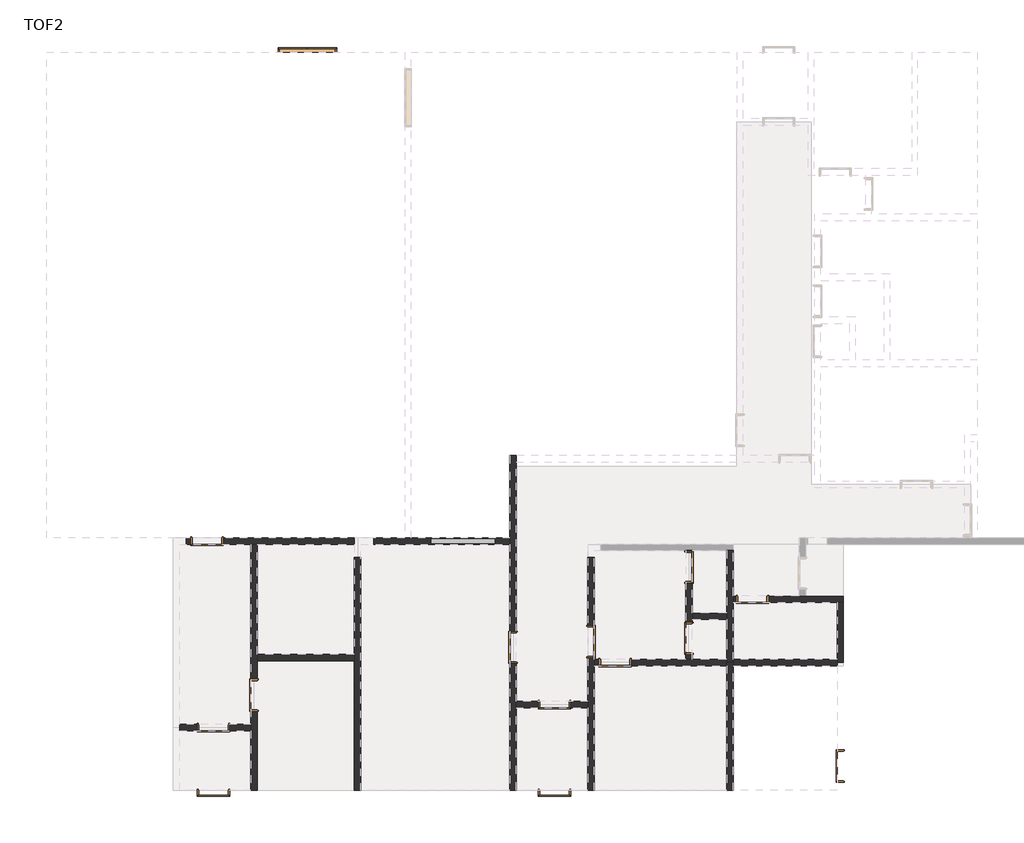
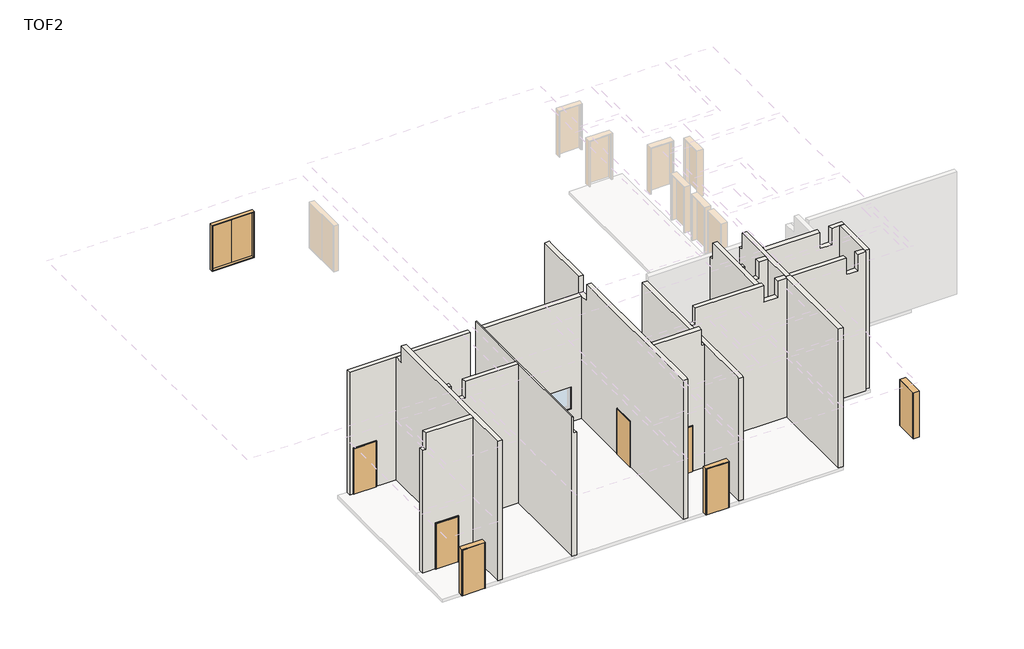
# One storey, part 1 of 2: 16 walls, 14 doors.
# Revit data of these elements (continued)
# Room at (25850, 15981.521) mm, phase "New Construction", upper level "TOC", upper offset 2000 mm, lower offset -2000 mm (continued)
#   H_Floor Finish Remark = "600x600, H=1000"
#   H_Skirt Base Material = "Same as Wall"
#   H_Skirt-Base Material-1 = ""
#   H_Skirt-Base Material-2 = ""
#   H_Skirt-Base Material-3 = ""
#   H_Skirt-Base Material-4 = ""
#   H_Skirt-Base Material-5 = ""
#   H_Skirt Finish-1 = "Vinyl Tile"
#   H_Skirt Finish-2 = ""
#   H_Skirt Finish Remark = "Vinyl Tile = PVC Tile (polyvinyl chloride)"
#   H_Wall Finish Style Name = "Acrylic Emulsion Paint"
#   H_Wall Base Material = "Masonry Wall / Cement Plaster"
#   H_Wall-Base Material-4 = ""
#   H_Wall-Base Material-5 = ""
#   H_Wall Finish-1 = "Acrylic Emulsion Paint"
#   H_Wall Finish-2 = ""
#   H_Wall Finish Remark = "T13 Plaster"
#   H_Ceiling Finish Style Name = "Suspended Acoustic Tiled Ceiling (M-Bar)"
#   H_Ceiling Base Material = "Concrete Slab / Fair Faced Concrete"
#   H_Ceiling-Base Material-1 = "(Concrete Slab)"
#   H_Ceiling-Base Material-2 = "(Fair Faced Concrete)"
#   H_Ceiling-Base Material-3 = ""
#   H_Ceiling-Base Material-4 = ""
#   H_Ceiling-Base Material-5 = "Acoustic Tiled Ceiling System (M-Bar)"
#   H_Ceiling Finish-1 = "Acoustic Tiled Ceiling System (M-Bar)"
#   H_Ceiling Finish-2 = ""
#   H_Ceiling Finish Remark = ""
#   Floor Finish Style No = F91
#   Skirt Finish Style No = B35
#   Wall Finish Style No = W01B
#   Ceiling Finish Style No = C95A
# Room at (22100, 4784.521) mm, phase "New Construction", upper level "TOC", upper offset 2000 mm, lower offset -2000 mm
#   Comments = ""
#   Number = "114"
#   Name = "BATTERY ROOM"
#   H_Floor Finish Style Name = "Acid Resistant Ceramic Tile"
#   H_Floor Base Material = "Concrete Slab / Steel Trowel Finish"
#   H_Wall-Base Material-1 = "Masonry Wall"
#   H_Skirt Finish Style Name = "Coved Vinyl Tile"
#   H_Wall-Base Material-2 = ""
#   H_Wall-Base Material-3 = "Plastering"
#   H_Floor-Base Material-1 = "Concrete Slab"
#   H_Floor-Base Material-2 = "Steel Trowel Finish"
#   H_Floor-Base Material-3 = ""
#   H_Floor-Base Material-4 = ""
#   H_Floor-Base Material-5 = "Acid/Alkaline Resistant Tile"
#   H_Floor Finish-1 = "Acid/Alkaline Resistant Tile"
#   H_Floor Finish-2 = ""
#   H_Floor Finish Remark = "*WM : Bonding용 Mortar은 Tile에 포함\n*Slope 용 Screed만 별도 구분 (Concrete 바닥 단차 발생하는 경우 Only)"
#   H_Skirt Base Material = "Same as Wall"
#   H_Skirt-Base Material-1 = ""
#   H_Skirt-Base Material-2 = ""
#   H_Skirt-Base Material-3 = ""
#   H_Skirt-Base Material-4 = ""
#   H_Skirt-Base Material-5 = ""
#   H_Skirt Finish-1 = "Vinyl Tile"
#   H_Skirt Finish-2 = ""
#   H_Skirt Finish Remark = "Vinyl Tile = PVC Tile (polyvinyl chloride)"
#   H_Wall Finish Style Name = "Acid Resistant Paint"
#   H_Wall Base Material = "Masonry Wall / Cement Plaster"
#   H_Wall-Base Material-4 = ""
#   H_Wall-Base Material-5 = ""
#   H_Wall Finish-1 = "Acid/Alkaline Resistant Paint"
#   H_Wall Finish-2 = ""
#   H_Wall Finish Remark = "T13 Plaster"
#   H_Ceiling Finish Style Name = "Acrylic Emulsion Paint"
#   H_Ceiling Base Material = "Concrete Slab / Fair Faced Concrete"
#   H_Ceiling-Base Material-1 = "(Concrete Slab)"
#   H_Ceiling-Base Material-2 = ""
#   H_Ceiling-Base Material-3 = ""
#   H_Ceiling-Base Material-4 = ""
#   H_Ceiling-Base Material-5 = ""
#   H_Ceiling Finish-1 = "Acrylic Emulsion Paint"
#   H_Ceiling Finish-2 = ""
#   H_Ceiling Finish Remark = "SACE"
#   Floor Finish Style No = F32A
#   Skirt Finish Style No = B35
#   Wall Finish Style No = W04B
#   Ceiling Finish Style No = C01
# Room at (34305, 4784.521) mm, phase "New Construction", upper level "TOC", upper offset 2000 mm, lower offset -2000 mm
#   Comments = ""
#   Number = "118"
#   Name = "DRIVERS LOUNGE"
#   H_Floor Finish Style Name = "Vinyl Tile"
#   H_Floor Base Material = "Concrete Slab / Steel Trowel Finish"
#   H_Wall-Base Material-1 = "Masonry Wall"
#   H_Skirt Finish Style Name = "Coved Vinyl Tile"
#   H_Wall-Base Material-2 = ""
#   H_Wall-Base Material-3 = "Plastering"
#   H_Floor-Base Material-1 = "Concrete Slab"
#   H_Floor-Base Material-2 = "Steel Trowel Finish"
#   H_Floor-Base Material-3 = ""
#   H_Floor-Base Material-4 = ""
#   H_Floor-Base Material-5 = "Vinyl Tile"
#   H_Floor Finish-1 = "Vinyl Tile"
#   H_Floor Finish-2 = ""
#   H_Floor Finish Remark = ""
#   H_Skirt Base Material = "Same as Wall"
#   H_Skirt-Base Material-1 = ""
#   H_Skirt-Base Material-2 = ""
#   H_Skirt-Base Material-3 = ""
#   H_Skirt-Base Material-4 = ""
#   H_Skirt-Base Material-5 = ""
#   H_Skirt Finish-1 = "Vinyl Tile"
#   H_Skirt Finish-2 = ""
#   H_Skirt Finish Remark = "Vinyl Tile = PVC Tile (polyvinyl chloride)"
#   H_Wall Finish Style Name = "Acrylic Emulsion Paint"
#   H_Wall Base Material = "Masonry Wall / Cement Plaster"
#   H_Wall-Base Material-4 = ""
#   H_Wall-Base Material-5 = ""
#   H_Wall Finish-1 = "Acrylic Emulsion Paint"
#   H_Wall Finish-2 = ""
#   H_Wall Finish Remark = "T13 Plaster"
#   H_Ceiling Finish Style Name = "Suspended Acoustic Tiled Ceiling (M-Bar)"
#   H_Ceiling Base Material = "Concrete Slab / Fair Faced Concrete"
#   H_Ceiling-Base Material-1 = "(Concrete Slab)"
#   H_Ceiling-Base Material-2 = "(Fair Faced Concrete)"
#   H_Ceiling-Base Material-3 = ""
#   H_Ceiling-Base Material-4 = ""
#   H_Ceiling-Base Material-5 = "Acoustic Tiled Ceiling System (M-Bar)"
#   H_Ceiling Finish-1 = "Acoustic Tiled Ceiling System (M-Bar)"
#   H_Ceiling Finish-2 = ""
#   H_Ceiling Finish Remark = ""
#   Floor Finish Style No = F34A
#   Skirt Finish Style No = B35
#   Wall Finish Style No = W01B
#   Ceiling Finish Style No = C95A
# Room at (38555, 16104.521) mm, phase "New Construction", upper level "TOC", upper offset 2000 mm, lower offset -2000 mm
#   Comments = ""
#   Number = "103"
#   Name = "CONTROL ROOM"
#   H_Floor Finish Style Name = "Anti-Dust Epoxy Paint / Anti-Static Vinyl Tile on Raised Floor"
#   H_Floor Base Material = "Concrete Slab / Steel Trowel Finish"
#   H_Wall-Base Material-1 = "Masonry Wall"
#   H_Skirt Finish Style Name = "Coved Vinyl Tile"
#   H_Wall-Base Material-2 = ""
#   H_Wall-Base Material-3 = "Plastering"
#   H_Floor-Base Material-1 = "Concrete Slab"
#   H_Floor-Base Material-2 = "Steel Trowel Finish"
#   H_Floor-Base Material-3 = ""
#   H_Floor-Base Material-4 = ""
#   H_Floor-Base Material-5 = "Raised Floor_Anti-Static Vinyl Tile"
#   H_Floor Finish-1 = "Anti-Dust Paint"
#   H_Floor Finish-2 = "Raised Floor_Anti-Static Vinyl Tile"
#   H_Floor Finish Remark = "600x600, H=1000"
#   H_Skirt Base Material = "Same as Wall"
#   H_Skirt-Base Material-1 = ""
#   H_Skirt-Base Material-2 = ""
#   H_Skirt-Base Material-3 = ""
#   H_Skirt-Base Material-4 = ""
#   H_Skirt-Base Material-5 = ""
#   H_Skirt Finish-1 = "Vinyl Tile"
#   H_Skirt Finish-2 = ""
#   H_Skirt Finish Remark = "Vinyl Tile = PVC Tile (polyvinyl chloride)"
#   H_Wall Finish Style Name = "Acrylic Emulsion Paint"
#   H_Wall Base Material = "Masonry Wall / Cement Plaster"
#   H_Wall-Base Material-4 = ""
#   H_Wall-Base Material-5 = ""
#   H_Wall Finish-1 = "Acrylic Emulsion Paint"
#   H_Wall Finish-2 = ""
#   H_Wall Finish Remark = "T13 Plaster"
#   H_Ceiling Finish Style Name = "Suspended Acoustic Tiled Ceiling (M-Bar)"
#   H_Ceiling Base Material = "Concrete Slab / Fair Faced Concrete"
#   H_Ceiling-Base Material-1 = "(Concrete Slab)"
#   H_Ceiling-Base Material-2 = "(Fair Faced Concrete)"
#   H_Ceiling-Base Material-3 = ""
#   H_Ceiling-Base Material-4 = ""
#   H_Ceiling-Base Material-5 = "Acoustic Tiled Ceiling System (M-Bar)"
#   H_Ceiling Finish-1 = "Acoustic Tiled Ceiling System (M-Bar)"
#   H_Ceiling Finish-2 = ""
#   H_Ceiling Finish Remark = ""
#   Floor Finish Style No = F91
#   Skirt Finish Style No = B35
#   Wall Finish Style No = W01B
#   Ceiling Finish Style No = C95A
# Room at (41150, 2419.673) mm, phase "New Construction", upper level "TOC", upper offset 2000 mm, lower offset -2000 mm
#   Comments = ""
#   Number = "122"
#   Name = "TOILETS"
#   H_Floor Finish Style Name = "Non-Slip Unglazed Ceramic Tile"
#   H_Floor Base Material = "Concrete Slab / Screed / Liquid Waterproofing"
#   H_Wall-Base Material-1 = "Masonry Wall"
#   H_Skirt Finish Style Name = "Coved Ceramic Tile"
#   H_Wall-Base Material-2 = ""
#   H_Wall-Base Material-3 = ""
#   H_Floor-Base Material-1 = "Concrete Slab"
#   H_Floor-Base Material-2 = ""
#   H_Floor-Base Material-3 = "Screed"
#   H_Floor-Base Material-4 = "Liquid Waterproofing"
#   H_Floor-Base Material-5 = "Ceramic Tile"
#   H_Floor Finish-1 = "Ceramic Tile"
#   H_Floor Finish-2 = ""
#   H_Floor Finish Remark = ""
#   H_Skirt Base Material = "Same as Wall"
#   H_Skirt-Base Material-1 = ""
#   H_Skirt-Base Material-2 = ""
#   H_Skirt-Base Material-3 = ""
#   H_Skirt-Base Material-4 = ""
#   H_Skirt-Base Material-5 = ""
#   H_Skirt Finish-1 = "Glazed Ceramic Tile"
#   H_Skirt Finish-2 = ""
#   H_Skirt Finish Remark = ""
#   H_Wall Finish Style Name = "Glazed Ceramic Tile (≤C.H+100) / No Paint (>C.H+100)"
#   H_Wall Base Material = "Masonry Wall / Liquid Waterproofing"
#   H_Wall-Base Material-4 = "Liquid Waterproofing"
#   H_Wall-Base Material-5 = "Glazed Ceramic Tile"
#   H_Wall Finish-1 = "Glazed Ceramic Tile"
#   H_Wall Finish-2 = ""
#   H_Wall Finish Remark = "Below Suspended Ceiling\nGlazed Ceramic Tile(≤C.H+100) + Liquid Waterproofing / No Paint (>C.H+100)"
#   H_Ceiling Finish Style Name = "Suspended Moisture Resistant Tiled Ceiling (M-Bar)"
#   H_Ceiling Base Material = "Concrete Slab / Fair Faced Concrete"
#   H_Ceiling-Base Material-1 = "(Concrete Slab)"
#   H_Ceiling-Base Material-2 = "(Fair Faced Concrete)"
#   H_Ceiling-Base Material-3 = ""
#   H_Ceiling-Base Material-4 = ""
#   H_Ceiling-Base Material-5 = "Moisture Resistant Tiled Ceiling System (M-Bar)"
#   H_Ceiling Finish-1 = "Moisture Resistant Tiled Ceiling System (M-Bar)"
#   H_Ceiling Finish-2 = ""
#   H_Ceiling Finish Remark = ""
#   Floor Finish Style No = F31B
#   Skirt Finish Style No = B32
#   Wall Finish Style No = W32B
#   Ceiling Finish Style No = C96A
# Room at (49742.5, 4429.521) mm, phase "New Construction", upper level "TOC", upper offset 2000 mm, lower offset -2000 mm
#   Comments = ""
#   Number = "125"
#   Name = "MAINTENANCE WORKSHOP"
#   H_Floor Finish Style Name = "Non-Slip Epoxy Paint"
#   H_Floor Base Material = "Concrete Slab / Steel Trowel Finish"
#   H_Wall-Base Material-1 = "Masonry Wall"
#   H_Skirt Finish Style Name = "Epoxy Paint"
#   H_Wall-Base Material-2 = ""
#   H_Wall-Base Material-3 = "Plastering"
#   H_Floor-Base Material-1 = "Concrete Slab"
#   H_Floor-Base Material-2 = "Steel Trowel Finish"
#   H_Floor-Base Material-3 = ""
#   H_Floor-Base Material-4 = ""
#   H_Floor-Base Material-5 = ""
#   H_Floor Finish-1 = "Epoxy Paint"
#   H_Floor Finish-2 = ""
#   H_Floor Finish Remark = "*WM 기준 확인 필요 Epoxy Paint \n(용제형, 0.1mm 이하) : epoxy resin + polyamine hardener(경화제)"
#   H_Skirt Base Material = "Same as Wall"
#   H_Skirt-Base Material-1 = ""
#   H_Skirt-Base Material-2 = ""
#   H_Skirt-Base Material-3 = ""
#   H_Skirt-Base Material-4 = ""
#   H_Skirt-Base Material-5 = ""
#   H_Skirt Finish-1 = "Epoxy Paint"
#   H_Skirt Finish-2 = ""
#   H_Skirt Finish Remark = "SACE"
#   H_Wall Finish Style Name = "Acrylic Emulsion Paint"
#   H_Wall Base Material = "Masonry Wall / Cement Plaster"
#   H_Wall-Base Material-4 = ""
#   H_Wall-Base Material-5 = ""
#   H_Wall Finish-1 = "Acrylic Emulsion Paint"
#   H_Wall Finish-2 = ""
#   H_Wall Finish Remark = "T13 Plaster"
#   H_Ceiling Finish Style Name = "Acrylic Emulsion Paint"
#   H_Ceiling Base Material = "Concrete Slab / Fair Faced Concrete"
#   H_Ceiling-Base Material-1 = "(Concrete Slab)"
#   H_Ceiling-Base Material-2 = ""
#   H_Ceiling-Base Material-3 = ""
#   H_Ceiling-Base Material-4 = ""
#   H_Ceiling-Base Material-5 = ""
#   H_Ceiling Finish-1 = "Acrylic Emulsion Paint"
#   H_Ceiling Finish-2 = ""
#   H_Ceiling Finish Remark = "SACE"
#   Floor Finish Style No = F06A
#   Skirt Finish Style No = B03
#   Wall Finish Style No = W01B
#   Ceiling Finish Style No = C01
# Room at (40470, 6702.369) mm, phase "New Construction", upper level "TOC", upper offset 2000 mm, lower offset -2000 mm
#   Comments = ""
#   Number = "121"
#   Name = "LOCKER"
#   H_Floor Finish Style Name = "Non-Slip Unglazed Ceramic Tile"
#   H_Floor Base Material = "Concrete Slab / Steel Trowel Finish"
#   H_Wall-Base Material-1 = "Masonry Wall"
#   H_Skirt Finish Style Name = "Coved Ceramic Tile"
#   H_Wall-Base Material-2 = ""
#   H_Wall-Base Material-3 = ""
#   H_Floor-Base Material-1 = "Concrete Slab"
#   H_Floor-Base Material-2 = "Steel Trowel Finish"
#   H_Floor-Base Material-3 = ""
#   H_Floor-Base Material-4 = ""
#   H_Floor-Base Material-5 = "Ceramic Tile"
#   H_Floor Finish-1 = "Ceramic Tile"
#   H_Floor Finish-2 = ""
#   H_Floor Finish Remark = "*WM : Bonding용 Mortar은 Tile에 포함\n*Slope 용 Screed만 별도 구분 (Concrete 바닥 단차 발생하는 경우 Only)"
#   H_Skirt Base Material = "Same as Wall"
#   H_Skirt-Base Material-1 = ""
#   H_Skirt-Base Material-2 = ""
#   H_Skirt-Base Material-3 = ""
#   H_Skirt-Base Material-4 = ""
#   H_Skirt-Base Material-5 = ""
#   H_Skirt Finish-1 = "Glazed Ceramic Tile"
#   H_Skirt Finish-2 = ""
#   H_Skirt Finish Remark = ""
#   H_Wall Finish Style Name = "Glazed Ceramic Tile (≤C.H+100) / No Paint (>C.H+100)"
#   H_Wall Base Material = "Masonry Wall / Liquid Waterproofing"
#   H_Wall-Base Material-4 = "Liquid Waterproofing"
#   H_Wall-Base Material-5 = "Glazed Ceramic Tile"
#   H_Wall Finish-1 = "Glazed Ceramic Tile"
#   H_Wall Finish-2 = ""
#   H_Wall Finish Remark = "Below Suspended Ceiling\nGlazed Ceramic Tile(≤C.H+100) + Liquid Waterproofing / No Paint (>C.H+100)"
#   H_Ceiling Finish Style Name = "Suspended Moisture Resistant Tiled Ceiling (M-Bar)"
#   H_Ceiling Base Material = "Concrete Slab / Fair Faced Concrete"
#   H_Ceiling-Base Material-1 = "(Concrete Slab)"
#   H_Ceiling-Base Material-2 = "(Fair Faced Concrete)"
#   H_Ceiling-Base Material-3 = ""
#   H_Ceiling-Base Material-4 = ""
#   H_Ceiling-Base Material-5 = "Moisture Resistant Tiled Ceiling System (M-Bar)"
#   H_Ceiling Finish-1 = "Moisture Resistant Tiled Ceiling System (M-Bar)"
#   H_Ceiling Finish-2 = ""
#   H_Ceiling Finish Remark = ""
#   Floor Finish Style No = F31A
#   Skirt Finish Style No = B32
#   Wall Finish Style No = W32B
#   Ceiling Finish Style No = C96A
# Room at (42630, 7074.521) mm, phase "New Construction", upper level "TOC", upper offset 2000 mm, lower offset -2000 mm
#   Comments = ""
#   Number = "127"
#   Name = "SHOWER ROOM"
#   H_Floor Finish Style Name = "Non-Slip Unglazed Ceramic Tile"
#   H_Floor Base Material = "Concrete Slab / Screed / Liquid Waterproofing"
#   H_Wall-Base Material-1 = "Concrete Wall"
#   H_Skirt Finish Style Name = "Epoxy Paint"
#   H_Wall-Base Material-2 = ""
#   H_Wall-Base Material-3 = ""
#   H_Floor-Base Material-1 = "Concrete Slab"
#   H_Floor-Base Material-2 = ""
#   H_Floor-Base Material-3 = "Screed"
#   H_Floor-Base Material-4 = "Liquid Waterproofing"
#   H_Floor-Base Material-5 = "Ceramic Tile"
#   H_Floor Finish-1 = "Ceramic Tile"
#   H_Floor Finish-2 = ""
#   H_Floor Finish Remark = ""
#   H_Skirt Base Material = "Same as Wall"
#   H_Skirt-Base Material-1 = ""
#   H_Skirt-Base Material-2 = ""
#   H_Skirt-Base Material-3 = ""
#   H_Skirt-Base Material-4 = ""
#   H_Skirt-Base Material-5 = ""
#   H_Skirt Finish-1 = "Epoxy Paint"
#   H_Skirt Finish-2 = ""
#   H_Skirt Finish Remark = "SACE"
#   H_Wall Finish Style Name = "Glazed Ceramic Tile (≤C.H+100) / No Paint (>C.H+100)"
#   H_Wall Base Material = "Concrete Wall"
#   H_Wall-Base Material-4 = "No Waterproofing"
#   H_Wall-Base Material-5 = "Glazed Ceramic Tile"
#   H_Wall Finish-1 = "Glazed Ceramic Tile"
#   H_Wall Finish-2 = ""
#   H_Wall Finish Remark = "Below Suspended Ceiling\nGlazed Ceramic Tile(≤C.H+100) / No Paint (>C.H+100)"
#   H_Ceiling Finish Style Name = "Suspended Moisture Resistant Tiled Ceiling (M-Bar)"
#   H_Ceiling Base Material = "Concrete Slab / Fair Faced Concrete"
#   H_Ceiling-Base Material-1 = "(Concrete Slab)"
#   H_Ceiling-Base Material-2 = "(Fair Faced Concrete)"
#   H_Ceiling-Base Material-3 = ""
#   H_Ceiling-Base Material-4 = ""
#   H_Ceiling-Base Material-5 = "Moisture Resistant Tiled Ceiling System (M-Bar)"
#   H_Ceiling Finish-1 = "Moisture Resistant Tiled Ceiling System (M-Bar)"
#   H_Ceiling Finish-2 = ""
#   H_Ceiling Finish Remark = ""
#   Floor Finish Style No = F31B
#   Skirt Finish Style No = B03
#   Wall Finish Style No = W32C
#   Ceiling Finish Style No = C96A
# Room at (42695, 5872.369) mm, phase "New Construction", upper level "TOC", upper offset 2000 mm, lower offset -2000 mm
#   Comments = ""
#   Number = "128"
#   Name = "EWH ROOM"
#   H_Floor Finish Style Name = "Non-Slip Unglazed Ceramic Tile"
#   H_Floor Base Material = "Concrete Slab / Steel Trowel Finish"
#   H_Wall-Base Material-1 = "Masonry Wall"
#   H_Skirt Finish Style Name = "Epoxy Paint"
#   H_Wall-Base Material-2 = ""
#   H_Wall-Base Material-3 = "Plastering"
#   H_Floor-Base Material-1 = "Concrete Slab"
#   H_Floor-Base Material-2 = "Steel Trowel Finish"
#   H_Floor-Base Material-3 = ""
#   H_Floor-Base Material-4 = ""
#   H_Floor-Base Material-5 = "Ceramic Tile"
#   H_Floor Finish-1 = "Ceramic Tile"
#   H_Floor Finish-2 = ""
#   H_Floor Finish Remark = "*WM : Bonding용 Mortar은 Tile에 포함\n*Slope 용 Screed만 별도 구분 (Concrete 바닥 단차 발생하는 경우 Only)"
#   H_Skirt Base Material = "Same as Wall"
#   H_Skirt-Base Material-1 = ""
#   H_Skirt-Base Material-2 = ""
#   H_Skirt-Base Material-3 = ""
#   H_Skirt-Base Material-4 = ""
#   H_Skirt-Base Material-5 = ""
#   H_Skirt Finish-1 = "Epoxy Paint"
#   H_Skirt Finish-2 = ""
#   H_Skirt Finish Remark = "SACE"
#   H_Wall Finish Style Name = "Acrylic Emulsion Paint"
#   H_Wall Base Material = "Masonry Wall / Cement Plaster"
#   H_Wall-Base Material-4 = ""
#   H_Wall-Base Material-5 = ""
#   H_Wall Finish-1 = "Acrylic Emulsion Paint"
#   H_Wall Finish-2 = ""
#   H_Wall Finish Remark = "T13 Plaster"
#   H_Ceiling Finish Style Name = "Suspended Acoustic Tiled Ceiling (M-Bar)"
#   H_Ceiling Base Material = "Concrete Slab / Fair Faced Concrete"
#   H_Ceiling-Base Material-1 = "(Concrete Slab)"
#   H_Ceiling-Base Material-2 = "(Fair Faced Concrete)"
#   H_Ceiling-Base Material-3 = ""
#   H_Ceiling-Base Material-4 = ""
#   H_Ceiling-Base Material-5 = "Acoustic Tiled Ceiling System (M-Bar)"
#   H_Ceiling Finish-1 = "Acoustic Tiled Ceiling System (M-Bar)"
#   H_Ceiling Finish-2 = ""
#   H_Ceiling Finish Remark = ""
#   Floor Finish Style No = F31A
#   Skirt Finish Style No = B03
#   Wall Finish Style No = W01B
#   Ceiling Finish Style No = C95A
# Room at (52032, 10149.521) mm, phase "New Construction", upper level "TOC", upper offset 2000 mm, lower offset -2000 mm
#   Comments = ""
#   Number = "110"
#   Name = "ABLUTIONS"
#   H_Floor Finish Style Name = "Non-Slip Unglazed Ceramic Tile"
#   H_Floor Base Material = "Concrete Slab / Screed / Liquid Waterproofing"
#   H_Wall-Base Material-1 = "Masonry Wall"
#   H_Skirt Finish Style Name = "Coved Ceramic Tile"
#   H_Wall-Base Material-2 = ""
#   H_Wall-Base Material-3 = ""
#   H_Floor-Base Material-1 = "Concrete Slab"
#   H_Floor-Base Material-2 = ""
#   H_Floor-Base Material-3 = "Screed"
#   H_Floor-Base Material-4 = "Liquid Waterproofing"
#   H_Floor-Base Material-5 = "Ceramic Tile"
#   H_Floor Finish-1 = "Ceramic Tile"
#   H_Floor Finish-2 = ""
#   H_Floor Finish Remark = ""
#   H_Skirt Base Material = "Same as Wall"
#   H_Skirt-Base Material-1 = ""
#   H_Skirt-Base Material-2 = ""
#   H_Skirt-Base Material-3 = ""
#   H_Skirt-Base Material-4 = ""
#   H_Skirt-Base Material-5 = ""
#   H_Skirt Finish-1 = "Glazed Ceramic Tile"
#   H_Skirt Finish-2 = ""
#   H_Skirt Finish Remark = ""
#   H_Wall Finish Style Name = "Glazed Ceramic Tile (≤C.H+100) / No Paint (>C.H+100)"
#   H_Wall Base Material = "Masonry Wall / Liquid Waterproofing"
#   H_Wall-Base Material-4 = "Liquid Waterproofing"
#   H_Wall-Base Material-5 = "Glazed Ceramic Tile"
#   H_Wall Finish-1 = "Glazed Ceramic Tile"
#   H_Wall Finish-2 = ""
#   H_Wall Finish Remark = "Below Suspended Ceiling\nGlazed Ceramic Tile(≤C.H+100) + Liquid Waterproofing / No Paint (>C.H+100)"
#   H_Ceiling Finish Style Name = "Suspended Moisture Resistant Tiled Ceiling (M-Bar)"
#   H_Ceiling Base Material = "Concrete Slab / Fair Faced Concrete"
#   H_Ceiling-Base Material-1 = "(Concrete Slab)"
#   H_Ceiling-Base Material-2 = "(Fair Faced Concrete)"
#   H_Ceiling-Base Material-3 = ""
#   H_Ceiling-Base Material-4 = ""
#   H_Ceiling-Base Material-5 = "Moisture Resistant Tiled Ceiling System (M-Bar)"
#   H_Ceiling Finish-1 = "Moisture Resistant Tiled Ceiling System (M-Bar)"
#   H_Ceiling Finish-2 = ""
#   H_Ceiling Finish Remark = ""
#   Floor Finish Style No = F31B
#   Skirt Finish Style No = B32
#   Wall Finish Style No = W32B
#   Ceiling Finish Style No = C96A
# Room at (50280, 21414.521) mm, phase "New Construction", upper level "TOC", upper offset 2000 mm, lower offset -2000 mm
#   Comments = ""
#   Number = "106"
#   Name = "SHIFT SUPERVISOR/DAY SUPERVISOR"
#   H_Floor Finish Style Name = "Vinyl Tile"
#   H_Floor Base Material = "Concrete Slab / Steel Trowel Finish"
#   H_Wall-Base Material-1 = "Masonry Wall"
#   H_Skirt Finish Style Name = "Coved Vinyl Tile"
#   H_Wall-Base Material-2 = ""
#   H_Wall-Base Material-3 = "Plastering"
#   H_Floor-Base Material-1 = "Concrete Slab"
#   H_Floor-Base Material-2 = "Steel Trowel Finish"
#   H_Floor-Base Material-3 = ""
#   H_Floor-Base Material-4 = ""
#   H_Floor-Base Material-5 = "Vinyl Tile"
#   H_Floor Finish-1 = "Vinyl Tile"
#   H_Floor Finish-2 = ""
#   H_Floor Finish Remark = ""
#   H_Skirt Base Material = "Same as Wall"
#   H_Skirt-Base Material-1 = ""
#   H_Skirt-Base Material-2 = ""
#   H_Skirt-Base Material-3 = ""
#   H_Skirt-Base Material-4 = ""
#   H_Skirt-Base Material-5 = ""
#   H_Skirt Finish-1 = "Vinyl Tile"
#   H_Skirt Finish-2 = ""
#   H_Skirt Finish Remark = "Vinyl Tile = PVC Tile (polyvinyl chloride)"
#   H_Wall Finish Style Name = "Acrylic Emulsion Paint"
#   H_Wall Base Material = "Masonry Wall / Cement Plaster"
#   H_Wall-Base Material-4 = ""
#   H_Wall-Base Material-5 = ""
#   H_Wall Finish-1 = "Acrylic Emulsion Paint"
#   H_Wall Finish-2 = ""
#   H_Wall Finish Remark = "T13 Plaster"
#   H_Ceiling Finish Style Name = "Suspended Acoustic Tiled Ceiling (M-Bar)"
#   H_Ceiling Base Material = "Concrete Slab / Fair Faced Concrete"
#   H_Ceiling-Base Material-1 = "(Concrete Slab)"
#   H_Ceiling-Base Material-2 = "(Fair Faced Concrete)"
#   H_Ceiling-Base Material-3 = ""
#   H_Ceiling-Base Material-4 = ""
#   H_Ceiling-Base Material-5 = "Acoustic Tiled Ceiling System (M-Bar)"
#   H_Ceiling Finish-1 = "Acoustic Tiled Ceiling System (M-Bar)"
#   H_Ceiling Finish-2 = ""
#   H_Ceiling Finish Remark = ""
#   Floor Finish Style No = F34A
#   Skirt Finish Style No = B35
#   Wall Finish Style No = W01B
#   Ceiling Finish Style No = C95A
# Room at (44795, 22494.021) mm, phase "New Construction", upper level "TOC", upper offset 2000 mm, lower offset -2000 mm
#   Comments = ""
#   Number = "104"
#   Name = "AIR LOCK"
#   H_Floor Finish Style Name = "Vinyl Tile"
#   H_Floor Base Material = "Concrete Slab / Steel Trowel Finish"
#   H_Wall-Base Material-1 = "Masonry Wall"
#   H_Skirt Finish Style Name = "Coved Vinyl Tile"
#   H_Wall-Base Material-2 = ""
#   H_Wall-Base Material-3 = "Plastering"
#   H_Floor-Base Material-1 = "Concrete Slab"
#   H_Floor-Base Material-2 = "Steel Trowel Finish"
#   H_Floor-Base Material-3 = ""
#   H_Floor-Base Material-4 = ""
#   H_Floor-Base Material-5 = "Vinyl Tile"
#   H_Floor Finish-1 = "Vinyl Tile"
#   H_Floor Finish-2 = ""
#   H_Floor Finish Remark = ""
#   H_Skirt Base Material = "Same as Wall"
#   H_Skirt-Base Material-1 = ""
#   H_Skirt-Base Material-2 = ""
#   H_Skirt-Base Material-3 = ""
#   H_Skirt-Base Material-4 = ""
#   H_Skirt-Base Material-5 = ""
#   H_Skirt Finish-1 = "Vinyl Tile"
#   H_Skirt Finish-2 = ""
#   H_Skirt Finish Remark = "Vinyl Tile = PVC Tile (polyvinyl chloride)"
#   H_Wall Finish Style Name = "Acrylic Emulsion Paint"
#   H_Wall Base Material = "Masonry Wall / Cement Plaster"
#   H_Wall-Base Material-4 = ""
#   H_Wall-Base Material-5 = ""
#   H_Wall Finish-1 = "Acrylic Emulsion Paint"
#   H_Wall Finish-2 = ""
#   H_Wall Finish Remark = "T13 Plaster"
#   H_Ceiling Finish Style Name = "Suspended Acoustic Tiled Ceiling (M-Bar)"
#   H_Ceiling Base Material = "Concrete Slab / Fair Faced Concrete"
#   H_Ceiling-Base Material-1 = "(Concrete Slab)"
#   H_Ceiling-Base Material-2 = "(Fair Faced Concrete)"
#   H_Ceiling-Base Material-3 = ""
#   H_Ceiling-Base Material-4 = ""
#   H_Ceiling-Base Material-5 = "Acoustic Tiled Ceiling System (M-Bar)"
#   H_Ceiling Finish-1 = "Acoustic Tiled Ceiling System (M-Bar)"
#   H_Ceiling Finish-2 = ""
#   H_Ceiling Finish Remark = ""
#   Floor Finish Style No = F34A
#   Skirt Finish Style No = B35
#   Wall Finish Style No = W01B
#   Ceiling Finish Style No = C95A
# Room at (45465, 16437.021) mm, phase "New Construction", upper level "TOC", upper offset 2000 mm, lower offset -2000 mm
#   Comments = ""
#   Number = "107"
#   Name = "CORRIDOR"
#   H_Floor Finish Style Name = "Vinyl Tile"
#   H_Floor Base Material = "Concrete Slab / Steel Trowel Finish"
#   H_Wall-Base Material-1 = "Masonry Wall"
#   H_Skirt Finish Style Name = "Coved Vinyl Tile"
#   H_Wall-Base Material-2 = ""
#   H_Wall-Base Material-3 = "Plastering"
#   H_Floor-Base Material-1 = "Concrete Slab"
#   H_Floor-Base Material-2 = "Steel Trowel Finish"
#   H_Floor-Base Material-3 = ""
#   H_Floor-Base Material-4 = ""
#   H_Floor-Base Material-5 = "Vinyl Tile"
#   H_Floor Finish-1 = "Vinyl Tile"
#   H_Floor Finish-2 = ""
#   H_Floor Finish Remark = ""
#   H_Skirt Base Material = "Same as Wall"
#   H_Skirt-Base Material-1 = ""
#   H_Skirt-Base Material-2 = ""
#   H_Skirt-Base Material-3 = ""
#   H_Skirt-Base Material-4 = ""
#   H_Skirt-Base Material-5 = ""
#   H_Skirt Finish-1 = "Vinyl Tile"
#   H_Skirt Finish-2 = ""
#   H_Skirt Finish Remark = "Vinyl Tile = PVC Tile (polyvinyl chloride)"
#   H_Wall Finish Style Name = "Acrylic Emulsion Paint"
#   H_Wall Base Material = "Masonry Wall / Cement Plaster"
#   H_Wall-Base Material-4 = ""
#   H_Wall-Base Material-5 = ""
#   H_Wall Finish-1 = "Acrylic Emulsion Paint"
#   H_Wall Finish-2 = ""
#   H_Wall Finish Remark = "T13 Plaster"
#   H_Ceiling Finish Style Name = "Suspended Acoustic Tiled Ceiling (M-Bar)"
#   H_Ceiling Base Material = "Concrete Slab / Fair Faced Concrete"
#   H_Ceiling-Base Material-1 = "(Concrete Slab)"
#   H_Ceiling-Base Material-2 = "(Fair Faced Concrete)"
#   H_Ceiling-Base Material-3 = ""
#   H_Ceiling-Base Material-4 = ""
#   H_Ceiling-Base Material-5 = "Acoustic Tiled Ceiling System (M-Bar)"
#   H_Ceiling Finish-1 = "Acoustic Tiled Ceiling System (M-Bar)"
#   H_Ceiling Finish-2 = ""
#   H_Ceiling Finish Remark = ""
#   Floor Finish Style No = F34A
#   Skirt Finish Style No = B35
#   Wall Finish Style No = W01B
#   Ceiling Finish Style No = C95A
# Room at (47300, 21676.521) mm, phase "New Construction", upper level "TOC", upper offset 2000 mm, lower offset -2000 mm
#   Comments = ""
#   Number = "105"
#   Name = "LIBRARY"
#   H_Floor Finish Style Name = "Vinyl Tile"
#   H_Floor Base Material = "Concrete Slab / Steel Trowel Finish"
#   H_Wall-Base Material-1 = "Masonry Wall"
#   H_Skirt Finish Style Name = "Coved Vinyl Tile"
#   H_Wall-Base Material-2 = ""
#   H_Wall-Base Material-3 = "Plastering"
#   H_Floor-Base Material-1 = "Concrete Slab"
#   H_Floor-Base Material-2 = "Steel Trowel Finish"
#   H_Floor-Base Material-3 = ""
#   H_Floor-Base Material-4 = ""
#   H_Floor-Base Material-5 = "Vinyl Tile"
#   H_Floor Finish-1 = "Vinyl Tile"
#   H_Floor Finish-2 = ""
#   H_Floor Finish Remark = ""
#   H_Skirt Base Material = "Same as Wall"
#   H_Skirt-Base Material-1 = ""
#   H_Skirt-Base Material-2 = ""
#   H_Skirt-Base Material-3 = ""
#   H_Skirt-Base Material-4 = ""
#   H_Skirt-Base Material-5 = ""
#   H_Skirt Finish-1 = "Vinyl Tile"
#   H_Skirt Finish-2 = ""
#   H_Skirt Finish Remark = "Vinyl Tile = PVC Tile (polyvinyl chloride)"
#   H_Wall Finish Style Name = "Acrylic Emulsion Paint"
#   H_Wall Base Material = "Masonry Wall / Cement Plaster"
#   H_Wall-Base Material-4 = ""
#   H_Wall-Base Material-5 = ""
#   H_Wall Finish-1 = "Acrylic Emulsion Paint"
#   H_Wall Finish-2 = ""
#   H_Wall Finish Remark = "T13 Plaster"
#   H_Ceiling Finish Style Name = "Suspended Acoustic Tiled Ceiling (M-Bar)"
#   H_Ceiling Base Material = "Concrete Slab / Fair Faced Concrete"
#   H_Ceiling-Base Material-1 = "(Concrete Slab)"
#   H_Ceiling-Base Material-2 = "(Fair Faced Concrete)"
#   H_Ceiling-Base Material-3 = ""
#   H_Ceiling-Base Material-4 = ""
#   H_Ceiling-Base Material-5 = "Acoustic Tiled Ceiling System (M-Bar)"
#   H_Ceiling Finish-1 = "Acoustic Tiled Ceiling System (M-Bar)"
#   H_Ceiling Finish-2 = ""
#   H_Ceiling Finish Remark = ""
#   Floor Finish Style No = F34A
#   Skirt Finish Style No = B35
#   Wall Finish Style No = W01B
#   Ceiling Finish Style No = C95A
# Room at (49372, 12124.521) mm, phase "New Construction", upper level "TOC", upper offset 2000 mm, lower offset -2000 mm
#   Comments = ""
#   Number = "111"
#   Name = "PRAYER ROOM"
#   H_Floor Finish Style Name = "Carpet Tile"
#   H_Floor Base Material = "Concrete Slab / Steel Trowel Finish"
#   H_Wall-Base Material-1 = "Masonry Wall"
#   H_Skirt Finish Style Name = "Coved Vinyl Tile"
#   H_Wall-Base Material-2 = ""
#   H_Wall-Base Material-3 = "Plastering"
#   H_Floor-Base Material-1 = "Concrete Slab"
#   H_Floor-Base Material-2 = ""
#   H_Floor-Base Material-3 = "Screed"
#   H_Floor-Base Material-5 = "Carpet Tile"
#   H_Floor Finish-1 = "Carpet Tile"
#   H_Skirt Base Material = "Same as Wall"
#   H_Skirt-Base Material-1 = ""
#   H_Skirt-Base Material-2 = ""
#   H_Skirt-Base Material-3 = ""
#   H_Skirt-Base Material-4 = ""
#   H_Skirt-Base Material-5 = ""
#   H_Skirt Finish-1 = "Vinyl Tile"
#   H_Skirt Finish-2 = ""
#   H_Skirt Finish Remark = "Vinyl Tile = PVC Tile (polyvinyl chloride)"
#   H_Wall Finish Style Name = "Acrylic Emulsion Paint"
#   H_Wall Base Material = "Masonry Wall / Cement Plaster"
#   H_Wall-Base Material-4 = ""
#   H_Wall-Base Material-5 = ""
#   H_Wall Finish-1 = "Acrylic Emulsion Paint"
#   H_Wall Finish-2 = ""
#   H_Wall Finish Remark = "T13 Plaster"
#   H_Ceiling Finish Style Name = "Suspended Acoustic Tiled Ceiling (M-Bar)"
#   H_Ceiling Base Material = "Concrete Slab / Fair Faced Concrete"
#   H_Ceiling-Base Material-1 = "(Concrete Slab)"
#   H_Ceiling-Base Material-2 = "(Fair Faced Concrete)"
#   H_Ceiling-Base Material-3 = ""
#   H_Ceiling-Base Material-4 = ""
#   H_Ceiling-Base Material-5 = "Acoustic Tiled Ceiling System (M-Bar)"
#   H_Ceiling Finish-1 = "Acoustic Tiled Ceiling System (M-Bar)"
#   H_Ceiling Finish-2 = ""
#   H_Ceiling Finish Remark = ""
#   Floor Finish Style No = F43-1
#   Skirt Finish Style No = B35
#   Wall Finish Style No = W01B
#   Ceiling Finish Style No = C95A
# Room at (49620, 16249.521) mm, phase "New Construction", upper level "TOC", upper offset 2000 mm, lower offset -2000 mm
#   Comments = ""
#   Number = "108"
#   Name = "BREAK ROOM"
#   H_Floor Finish Style Name = "Vinyl Tile"
#   H_Floor Base Material = "Concrete Slab / Steel Trowel Finish"
#   H_Wall-Base Material-1 = "Masonry Wall"
#   H_Skirt Finish Style Name = "Coved Vinyl Tile"
#   H_Wall-Base Material-2 = ""
#   H_Wall-Base Material-3 = "Plastering"
#   H_Floor-Base Material-1 = "Concrete Slab"
#   H_Floor-Base Material-2 = "Steel Trowel Finish"
#   H_Floor-Base Material-3 = ""
#   H_Floor-Base Material-4 = ""
#   H_Floor-Base Material-5 = "Vinyl Tile"
#   H_Floor Finish-1 = "Vinyl Tile"
#   H_Floor Finish-2 = ""
#   H_Floor Finish Remark = ""
#   H_Skirt Base Material = "Same as Wall"
#   H_Skirt-Base Material-1 = ""
#   H_Skirt-Base Material-2 = ""
#   H_Skirt-Base Material-3 = ""
#   H_Skirt-Base Material-4 = ""
#   H_Skirt-Base Material-5 = ""
#   H_Skirt Finish-1 = "Vinyl Tile"
#   H_Skirt Finish-2 = ""
#   H_Skirt Finish Remark = "Vinyl Tile = PVC Tile (polyvinyl chloride)"
#   H_Wall Finish Style Name = "Acrylic Emulsion Paint"
#   H_Wall Base Material = "Masonry Wall / Cement Plaster"
#   H_Wall-Base Material-4 = ""
#   H_Wall-Base Material-5 = ""
#   H_Wall Finish-1 = "Acrylic Emulsion Paint"
#   H_Wall Finish-2 = ""
#   H_Wall Finish Remark = "T13 Plaster"
#   H_Ceiling Finish Style Name = "Suspended Moisture Resistant Tiled Ceiling (M-Bar)"
#   H_Ceiling Base Material = "Concrete Slab / Fair Faced Concrete"
#   H_Ceiling-Base Material-1 = "(Concrete Slab)"
#   H_Ceiling-Base Material-2 = "(Fair Faced Concrete)"
#   H_Ceiling-Base Material-3 = ""
#   H_Ceiling-Base Material-4 = ""
#   H_Ceiling-Base Material-5 = "Moisture Resistant Tiled Ceiling System (M-Bar)"
#   H_Ceiling Finish-1 = "Moisture Resistant Tiled Ceiling System (M-Bar)"
#   H_Ceiling Finish-2 = ""
#   H_Ceiling Finish Remark = ""
#   Floor Finish Style No = F34A
#   Skirt Finish Style No = B35
#   Wall Finish Style No = W01B
#   Ceiling Finish Style No = C96A
# Room at (47117.5, 15324.521) mm, phase "New Construction", upper level "TOC", upper offset 2000 mm, lower offset -2000 mm
#   Comments = ""
#   Number = "109"
#   Name = "JANITOR"
#   H_Floor Finish Style Name = "Non-Slip Unglazed Ceramic Tile"
#   H_Floor Base Material = "Concrete Slab / Screed / Liquid Waterproofing"
#   H_Wall-Base Material-1 = "Masonry Wall"
#   H_Skirt Finish Style Name = "Coved Ceramic Tile"
#   H_Wall-Base Material-2 = ""
#   H_Wall-Base Material-3 = ""
#   H_Floor-Base Material-1 = "Concrete Slab"
#   H_Floor-Base Material-2 = ""
#   H_Floor-Base Material-3 = "Screed"
#   H_Floor-Base Material-4 = "Liquid Waterproofing"
#   H_Floor-Base Material-5 = "Ceramic Tile"
#   H_Floor Finish-1 = "Ceramic Tile"
#   H_Floor Finish-2 = ""
#   H_Floor Finish Remark = ""
#   H_Skirt Base Material = "Same as Wall"
#   H_Skirt-Base Material-1 = ""
#   H_Skirt-Base Material-2 = ""
#   H_Skirt-Base Material-3 = ""
#   H_Skirt-Base Material-4 = ""
#   H_Skirt-Base Material-5 = ""
#   H_Skirt Finish-1 = "Glazed Ceramic Tile"
#   H_Skirt Finish-2 = ""
#   H_Skirt Finish Remark = ""
#   H_Wall Finish Style Name = "Glazed Ceramic Tile (≤C.H+100) / No Paint (>C.H+100)"
#   H_Wall Base Material = "Masonry Wall / Liquid Waterproofing"
#   H_Wall-Base Material-4 = "Liquid Waterproofing"
#   H_Wall-Base Material-5 = "Glazed Ceramic Tile"
#   H_Wall Finish-1 = "Glazed Ceramic Tile"
#   H_Wall Finish-2 = ""
#   H_Wall Finish Remark = "Below Suspended Ceiling\nGlazed Ceramic Tile(≤C.H+100) + Liquid Waterproofing / No Paint (>C.H+100)"
#   H_Ceiling Finish Style Name = "Suspended Moisture Resistant Tiled Ceiling (M-Bar)"
#   H_Ceiling Base Material = "Concrete Slab / Fair Faced Concrete"
#   H_Ceiling-Base Material-1 = "(Concrete Slab)"
#   H_Ceiling-Base Material-2 = "(Fair Faced Concrete)"
#   H_Ceiling-Base Material-3 = ""
#   H_Ceiling-Base Material-4 = ""
#   H_Ceiling-Base Material-5 = "Moisture Resistant Tiled Ceiling System (M-Bar)"
#   H_Ceiling Finish-1 = "Moisture Resistant Tiled Ceiling System (M-Bar)"
#   H_Ceiling Finish-2 = ""
#   H_Ceiling Finish Remark = ""
#   Floor Finish Style No = F31B
#   Skirt Finish Style No = B32
#   Wall Finish Style No = W32B
#   Ceiling Finish Style No = C96A
# Room at (46580, 14657.021) mm, phase "New Construction", upper level "TOC", upper offset 2000 mm, lower offset -2000 mm
#   Comments = ""
#   Number = "126"
#   Name = "EWH ROOM"
#   H_Floor Finish Style Name = "Vinyl Tile"
#   H_Floor Base Material = "Concrete Slab / Steel Trowel Finish"
#   H_Wall-Base Material-1 = "Masonry Wall"
#   H_Skirt Finish Style Name = "Coved Vinyl Tile"
#   H_Wall-Base Material-2 = ""
#   H_Wall-Base Material-3 = "Plastering"
#   H_Floor-Base Material-1 = "Concrete Slab"
#   H_Floor-Base Material-2 = "Steel Trowel Finish"
#   H_Floor-Base Material-3 = ""
#   H_Floor-Base Material-4 = ""
#   H_Floor-Base Material-5 = "Vinyl Tile"
#   H_Floor Finish-1 = "Vinyl Tile"
#   H_Floor Finish-2 = ""
#   H_Floor Finish Remark = ""
#   H_Skirt Base Material = "Same as Wall"
#   H_Skirt-Base Material-1 = ""
#   H_Skirt-Base Material-2 = ""
#   H_Skirt-Base Material-3 = ""
#   H_Skirt-Base Material-4 = ""
#   H_Skirt-Base Material-5 = ""
#   H_Skirt Finish-1 = "Vinyl Tile"
#   H_Skirt Finish-2 = ""
#   H_Skirt Finish Remark = "Vinyl Tile = PVC Tile (polyvinyl chloride)"
#   H_Wall Finish Style Name = "Acrylic Emulsion Paint"
#   H_Wall Base Material = "Masonry Wall / Cement Plaster"
#   H_Wall-Base Material-4 = ""
#   H_Wall-Base Material-5 = ""
#   H_Wall Finish-1 = "Acrylic Emulsion Paint"
#   H_Wall Finish-2 = ""
#   H_Wall Finish Remark = "T13 Plaster"
#   H_Ceiling Finish Style Name = "Suspended Acoustic Tiled Ceiling (M-Bar)"
#   H_Ceiling Base Material = "Concrete Slab / Fair Faced Concrete"
#   H_Ceiling-Base Material-1 = "(Concrete Slab)"
#   H_Ceiling-Base Material-2 = "(Fair Faced Concrete)"
#   H_Ceiling-Base Material-3 = ""
#   H_Ceiling-Base Material-4 = ""
#   H_Ceiling-Base Material-5 = "Acoustic Tiled Ceiling System (M-Bar)"
#   H_Ceiling Finish-1 = "Acoustic Tiled Ceiling System (M-Bar)"
#   H_Ceiling Finish-2 = ""
#   H_Ceiling Finish Remark = ""
#   Floor Finish Style No = F34A
#   Skirt Finish Style No = B35
#   Wall Finish Style No = W01B
#   Ceiling Finish Style No = C95A
# Room at (45350, 5729.521) mm, phase "New Construction", upper level "TOC", upper offset 2000 mm, lower offset -2000 mm
#   Comments = ""
#   Number = "123"
#   Name = "STORE"
#   H_Floor Finish Style Name = "Vinyl Tile"
#   H_Floor Base Material = "Concrete Slab / Steel Trowel Finish"
#   H_Wall-Base Material-1 = "Masonry Wall"
#   H_Skirt Finish Style Name = "Coved Vinyl Tile"
#   H_Wall-Base Material-2 = ""
#   H_Wall-Base Material-3 = "Plastering"
#   H_Floor-Base Material-1 = "Concrete Slab"
#   H_Floor-Base Material-2 = "Steel Trowel Finish"
#   H_Floor-Base Material-3 = ""
#   H_Floor-Base Material-4 = ""
#   H_Floor-Base Material-5 = "Vinyl Tile"
#   H_Floor Finish-1 = "Vinyl Tile"
#   H_Floor Finish-2 = ""
#   H_Floor Finish Remark = ""
#   H_Skirt Base Material = "Same as Wall"
#   H_Skirt-Base Material-1 = ""
#   H_Skirt-Base Material-2 = ""
#   H_Skirt-Base Material-3 = ""
#   H_Skirt-Base Material-4 = ""
#   H_Skirt-Base Material-5 = ""
#   H_Skirt Finish-1 = "Vinyl Tile"
#   H_Skirt Finish-2 = ""
#   H_Skirt Finish Remark = "Vinyl Tile = PVC Tile (polyvinyl chloride)"
#   H_Wall Finish Style Name = "Acrylic Emulsion Paint"
#   H_Wall Base Material = "Masonry Wall / Cement Plaster"
#   H_Wall-Base Material-4 = ""
#   H_Wall-Base Material-5 = ""
#   H_Wall Finish-1 = "Acrylic Emulsion Paint"
#   H_Wall Finish-2 = ""
#   H_Wall Finish Remark = "T13 Plaster"
#   H_Ceiling Finish Style Name = "Suspended Acoustic Tiled Ceiling (M-Bar)"
#   H_Ceiling Base Material = "Concrete Slab / Fair Faced Concrete"
#   H_Ceiling-Base Material-1 = "(Concrete Slab)"
#   H_Ceiling-Base Material-2 = "(Fair Faced Concrete)"
#   H_Ceiling-Base Material-3 = ""
#   H_Ceiling-Base Material-4 = ""
#   H_Ceiling-Base Material-5 = "Acoustic Tiled Ceiling System (M-Bar)"
#   H_Ceiling Finish-1 = "Acoustic Tiled Ceiling System (M-Bar)"
#   H_Ceiling Finish-2 = ""
#   H_Ceiling Finish Remark = ""
#   Floor Finish Style No = F34A
#   Skirt Finish Style No = B35
#   Wall Finish Style No = W01B
#   Ceiling Finish Style No = C95A
# Room at (45350, 2414.673) mm, phase "New Construction", upper level "TOC", upper offset 2000 mm, lower offset -2000 mm
#   Comments = ""
#   Number = "124"
#   Name = "STORE"
#   H_Floor Finish Style Name = "Vinyl Tile"
#   H_Floor Base Material = "Concrete Slab / Steel Trowel Finish"
#   H_Wall-Base Material-1 = "Masonry Wall"
#   H_Skirt Finish Style Name = "Coved Vinyl Tile"
#   H_Wall-Base Material-2 = ""
#   H_Wall-Base Material-3 = "Plastering"
#   H_Floor-Base Material-1 = "Concrete Slab"
#   H_Floor-Base Material-2 = "Steel Trowel Finish"
#   H_Floor-Base Material-3 = ""
#   H_Floor-Base Material-4 = ""
#   H_Floor-Base Material-5 = "Vinyl Tile"
#   H_Floor Finish-1 = "Vinyl Tile"
#   H_Floor Finish-2 = ""
#   H_Floor Finish Remark = ""
#   H_Skirt Base Material = "Same as Wall"
#   H_Skirt-Base Material-1 = ""
#   H_Skirt-Base Material-2 = ""
#   H_Skirt-Base Material-3 = ""
#   H_Skirt-Base Material-4 = ""
#   H_Skirt-Base Material-5 = ""
#   H_Skirt Finish-1 = "Vinyl Tile"
#   H_Skirt Finish-2 = ""
#   H_Skirt Finish Remark = "Vinyl Tile = PVC Tile (polyvinyl chloride)"
#   H_Wall Finish Style Name = "Acrylic Emulsion Paint"
#   H_Wall Base Material = "Masonry Wall / Cement Plaster"
#   H_Wall-Base Material-4 = ""
#   H_Wall-Base Material-5 = ""
#   H_Wall Finish-1 = "Acrylic Emulsion Paint"
#   H_Wall Finish-2 = ""
#   H_Wall Finish Remark = "T13 Plaster"
#   H_Ceiling Finish Style Name = "Suspended Acoustic Tiled Ceiling (M-Bar)"
#   H_Ceiling Base Material = "Concrete Slab / Fair Faced Concrete"
#   H_Ceiling-Base Material-1 = "(Concrete Slab)"
#   H_Ceiling-Base Material-2 = "(Fair Faced Concrete)"
#   H_Ceiling-Base Material-3 = ""
#   H_Ceiling-Base Material-4 = ""
#   H_Ceiling-Base Material-5 = "Acoustic Tiled Ceiling System (M-Bar)"
#   H_Ceiling Finish-1 = "Acoustic Tiled Ceiling System (M-Bar)"
#   H_Ceiling Finish-2 = ""
#   H_Ceiling Finish Remark = ""
#   Floor Finish Style No = F34A
#   Skirt Finish Style No = B35
#   Wall Finish Style No = W01B
#   Ceiling Finish Style No = C95A
# Room at (30342.5, 2466.271) mm, phase "New Construction", upper level "TOC", upper offset 2000 mm, lower offset -2000 mm
#   Comments = ""
#   Number = "115"
#   Name = "TELECOMS ROOM"
#   H_Floor Finish Style Name = "Vinyl Tile"
#   H_Floor Base Material = "Concrete Slab / Steel Trowel Finish"
#   H_Wall-Base Material-1 = "Concrete Wall"
#   H_Skirt Finish Style Name = "Coved Vinyl Tile"
#   H_Wall-Base Material-2 = "(Fair Faced Concrete)"
#   H_Wall-Base Material-3 = ""
#   H_Floor-Base Material-1 = "Concrete Slab"
#   H_Floor-Base Material-2 = "Steel Trowel Finish"
#   H_Floor-Base Material-3 = ""
#   H_Floor-Base Material-4 = ""
#   H_Floor-Base Material-5 = "Vinyl Tile"
#   H_Floor Finish-1 = "Vinyl Tile"
#   H_Floor Finish-2 = ""
#   H_Floor Finish Remark = ""
#   H_Skirt Base Material = "Same as Wall"
#   H_Skirt-Base Material-1 = ""
#   H_Skirt-Base Material-2 = ""
#   H_Skirt-Base Material-3 = ""
#   H_Skirt-Base Material-4 = ""
#   H_Skirt-Base Material-5 = ""
#   H_Skirt Finish-1 = "Vinyl Tile"
#   H_Skirt Finish-2 = ""
#   H_Skirt Finish Remark = "Vinyl Tile = PVC Tile (polyvinyl chloride)"
#   H_Wall Finish Style Name = "Latex Paint"
#   H_Wall Base Material = "Concrete Wall / Fair Faced Concrete"
#   H_Wall-Base Material-4 = ""
#   H_Wall-Base Material-5 = ""
#   H_Wall Finish-1 = "Latex Paint"
#   H_Wall Finish-2 = ""
#   H_Wall Finish Remark = ""
#   H_Ceiling Finish Style Name = "Acrylic Emulsion Paint"
#   H_Ceiling Base Material = "Concrete Slab / Fair Faced Concrete"
#   H_Ceiling-Base Material-1 = "(Concrete Slab)"
#   H_Ceiling-Base Material-2 = ""
#   H_Ceiling-Base Material-3 = ""
#   H_Ceiling-Base Material-4 = ""
#   H_Ceiling-Base Material-5 = ""
#   H_Ceiling Finish-1 = "Acrylic Emulsion Paint"
#   H_Ceiling Finish-2 = ""
#   H_Ceiling Finish Remark = "SACE"
#   Floor Finish Style No = F34A
#   Skirt Finish Style No = B35
#   Wall Finish Style No = W03A
#   Ceiling Finish Style No = C01
# Room at (30057.5, 6598.271) mm, phase "New Construction", upper level "TOC", upper offset 2000 mm, lower offset -2000 mm
#   Comments = ""
#   Number = "113"
#   Name = "STORE"
#   H_Floor Finish Style Name = "Vinyl Tile"
#   H_Floor Base Material = "Concrete Slab / Steel Trowel Finish"
#   H_Wall-Base Material-1 = "Masonry Wall"
#   H_Skirt Finish Style Name = "Coved Vinyl Tile"
#   H_Wall-Base Material-2 = ""
#   H_Wall-Base Material-3 = "Plastering"
#   H_Floor-Base Material-1 = "Concrete Slab"
#   H_Floor-Base Material-2 = "Steel Trowel Finish"
#   H_Floor-Base Material-3 = ""
#   H_Floor-Base Material-4 = ""
#   H_Floor-Base Material-5 = "Vinyl Tile"
#   H_Floor Finish-1 = "Vinyl Tile"
#   H_Floor Finish-2 = ""
#   H_Floor Finish Remark = ""
#   H_Skirt Base Material = "Same as Wall"
#   H_Skirt-Base Material-1 = ""
#   H_Skirt-Base Material-2 = ""
#   H_Skirt-Base Material-3 = ""
#   H_Skirt-Base Material-4 = ""
#   H_Skirt-Base Material-5 = ""
#   H_Skirt Finish-1 = "Vinyl Tile"
#   H_Skirt Finish-2 = ""
#   H_Skirt Finish Remark = "Vinyl Tile = PVC Tile (polyvinyl chloride)"
#   H_Wall Finish Style Name = "Acrylic Emulsion Paint"
#   H_Wall Base Material = "Masonry Wall / Cement Plaster"
#   H_Wall-Base Material-4 = ""
#   H_Wall-Base Material-5 = ""
#   H_Wall Finish-1 = "Acrylic Emulsion Paint"
#   H_Wall Finish-2 = ""
#   H_Wall Finish Remark = "T13 Plaster"
#   H_Ceiling Finish Style Name = "Suspended Acoustic Tiled Ceiling (M-Bar)"
#   H_Ceiling Base Material = "Concrete Slab / Fair Faced Concrete"
#   H_Ceiling-Base Material-1 = "(Concrete Slab)"
#   H_Ceiling-Base Material-2 = "(Fair Faced Concrete)"
#   H_Ceiling-Base Material-3 = ""
#   H_Ceiling-Base Material-4 = ""
#   H_Ceiling-Base Material-5 = "Acoustic Tiled Ceiling System (M-Bar)"
#   H_Ceiling Finish-1 = "Acoustic Tiled Ceiling System (M-Bar)"
#   H_Ceiling Finish-2 = ""
#   H_Ceiling Finish Remark = ""
#   Floor Finish Style No = F34A
#   Skirt Finish Style No = B35
#   Wall Finish Style No = W01B
#   Ceiling Finish Style No = C95A
# Room at (27362.5, 1628.771) mm, phase "New Construction", upper level "TOC", upper offset 2000 mm, lower offset -2000 mm
#   Comments = ""
#   Number = "117"
#   Name = "AIR LOCK"
#   H_Floor Finish Style Name = "Vinyl Tile"
#   H_Floor Base Material = "Concrete Slab / Steel Trowel Finish"
#   H_Wall-Base Material-1 = "Masonry Wall"
#   H_Skirt Finish Style Name = "Coved Vinyl Tile"
#   H_Wall-Base Material-2 = ""
#   H_Wall-Base Material-3 = "Plastering"
#   H_Floor-Base Material-1 = "Concrete Slab"
#   H_Floor-Base Material-2 = "Steel Trowel Finish"
#   H_Floor-Base Material-3 = ""
#   H_Floor-Base Material-4 = ""
#   H_Floor-Base Material-5 = "Vinyl Tile"
#   H_Floor Finish-1 = "Vinyl Tile"
#   H_Floor Finish-2 = ""
#   H_Floor Finish Remark = ""
#   H_Skirt Base Material = "Same as Wall"
#   H_Skirt-Base Material-1 = ""
#   H_Skirt-Base Material-2 = ""
#   H_Skirt-Base Material-3 = ""
#   H_Skirt-Base Material-4 = ""
#   H_Skirt-Base Material-5 = ""
#   H_Skirt Finish-1 = "Vinyl Tile"
#   H_Skirt Finish-2 = ""
#   H_Skirt Finish Remark = "Vinyl Tile = PVC Tile (polyvinyl chloride)"
#   H_Wall Finish Style Name = "Acrylic Emulsion Paint"
#   H_Wall Base Material = "Masonry Wall / Cement Plaster"
#   H_Wall-Base Material-4 = ""
#   H_Wall-Base Material-5 = ""
#   H_Wall Finish-1 = "Acrylic Emulsion Paint"
#   H_Wall Finish-2 = ""
#   H_Wall Finish Remark = "T13 Plaster"
#   H_Ceiling Finish Style Name = "Suspended Acoustic Tiled Ceiling (M-Bar)"
#   H_Ceiling Base Material = "Concrete Slab / Fair Faced Concrete"
#   H_Ceiling-Base Material-1 = "(Concrete Slab)"
#   H_Ceiling-Base Material-2 = "(Fair Faced Concrete)"
#   H_Ceiling-Base Material-3 = ""
#   H_Ceiling-Base Material-4 = ""
#   H_Ceiling-Base Material-5 = "Acoustic Tiled Ceiling System (M-Bar)"
#   H_Ceiling Finish-1 = "Acoustic Tiled Ceiling System (M-Bar)"
#   H_Ceiling Finish-2 = ""
#   H_Ceiling Finish Remark = ""
#   Floor Finish Style No = F34A
#   Skirt Finish Style No = B35
#   Wall Finish Style No = W01B
#   Ceiling Finish Style No = C95A
# Room at (27362.5, 5760.771) mm, phase "New Construction", upper level "TOC", upper offset 2000 mm, lower offset -2000 mm
#   Comments = ""
#   Number = "116"
#   Name = "CORRIDOR"
#   H_Floor Finish Style Name = "Vinyl Tile"
#   H_Floor Base Material = "Concrete Slab / Steel Trowel Finish"
#   H_Wall-Base Material-1 = "Masonry Wall"
#   H_Skirt Finish Style Name = "Coved Vinyl Tile"
#   H_Wall-Base Material-2 = ""
#   H_Wall-Base Material-3 = "Plastering"
#   H_Floor-Base Material-1 = "Concrete Slab"
#   H_Floor-Base Material-2 = "Steel Trowel Finish"
#   H_Floor-Base Material-3 = ""
#   H_Floor-Base Material-4 = ""
#   H_Floor-Base Material-5 = "Vinyl Tile"
#   H_Floor Finish-1 = "Vinyl Tile"
#   H_Floor Finish-2 = ""
#   H_Floor Finish Remark = ""
#   H_Skirt Base Material = "Same as Wall"
#   H_Skirt-Base Material-1 = ""
#   H_Skirt-Base Material-2 = ""
#   H_Skirt-Base Material-3 = ""
#   H_Skirt-Base Material-4 = ""
#   H_Skirt-Base Material-5 = ""
#   H_Skirt Finish-1 = "Vinyl Tile"
#   H_Skirt Finish-2 = ""
#   H_Skirt Finish Remark = "Vinyl Tile = PVC Tile (polyvinyl chloride)"
#   H_Wall Finish Style Name = "Acrylic Emulsion Paint"
#   H_Wall Base Material = "Masonry Wall / Cement Plaster"
#   H_Wall-Base Material-4 = ""
#   H_Wall-Base Material-5 = ""
#   H_Wall Finish-1 = "Acrylic Emulsion Paint"
#   H_Wall Finish-2 = ""
#   H_Wall Finish Remark = "T13 Plaster"
#   H_Ceiling Finish Style Name = "Suspended Acoustic Tiled Ceiling (M-Bar)"
#   H_Ceiling Base Material = "Concrete Slab / Fair Faced Concrete"
#   H_Ceiling-Base Material-1 = "(Concrete Slab)"
#   H_Ceiling-Base Material-2 = "(Fair Faced Concrete)"
#   H_Ceiling-Base Material-3 = ""
#   H_Ceiling-Base Material-4 = ""
#   H_Ceiling-Base Material-5 = "Acoustic Tiled Ceiling System (M-Bar)"
#   H_Ceiling Finish-1 = "Acoustic Tiled Ceiling System (M-Bar)"
#   H_Ceiling Finish-2 = ""
#   H_Ceiling Finish Remark = ""
#   Floor Finish Style No = F34A
#   Skirt Finish Style No = B35
#   Wall Finish Style No = W01B
#   Ceiling Finish Style No = C95A
# Room at (43870, 7604.869) mm, phase "New Construction", upper level "TOC", upper offset 2000 mm, lower offset -2000 mm
#   Comments = ""
#   Number = "120"
#   Name = "CORRIDOR"
#   H_Floor Finish Style Name = "Vinyl Tile"
#   H_Floor Base Material = "Concrete Slab / Steel Trowel Finish"
#   H_Wall-Base Material-1 = "Masonry Wall"
#   H_Skirt Finish Style Name = "Coved Vinyl Tile"
#   H_Wall-Base Material-2 = ""
#   H_Wall-Base Material-3 = "Plastering"
#   H_Floor-Base Material-1 = "Concrete Slab"
